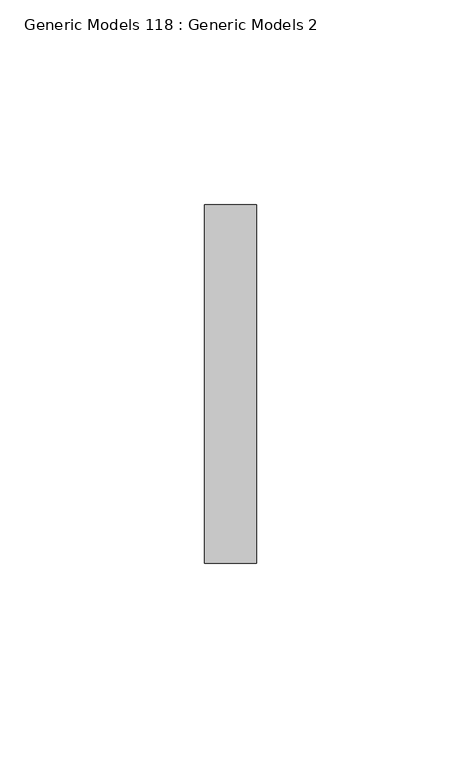
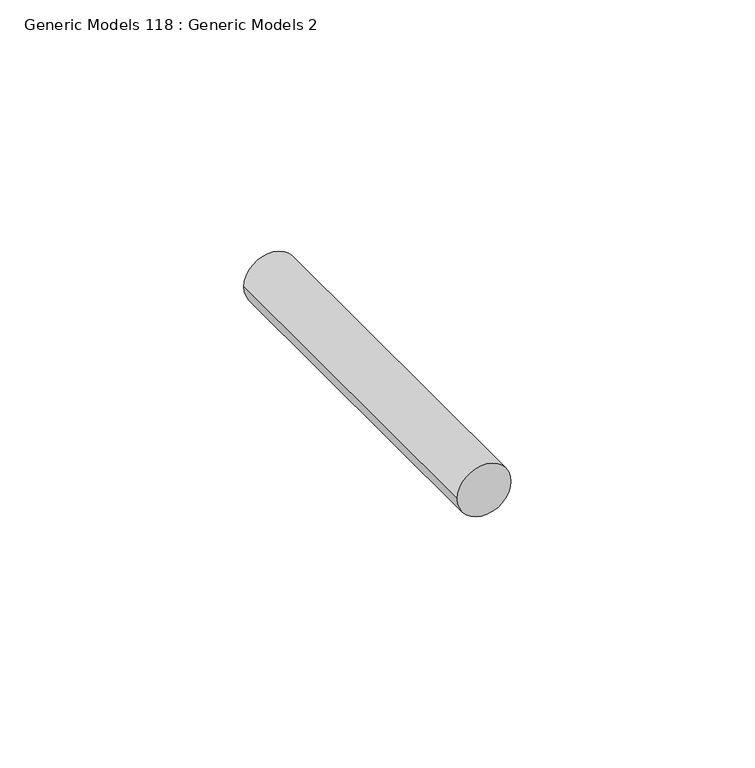
"""IFC4 building model written with IfcOpenShell, lengths in millimetres: proxy geometry, Generic Models 118 : Generic Models 2."""

from ifc_helpers import new_model, si_unit, point, frame, frame_2d, origin, place, context, project, spatial, circle_curve, trimmed, segment, composite_curve, outline, extrude, source, transform, mapped, element, save


def generic_models_118_generic_models_2_6a2263a1(model_context):
    return source(origin(), model_context, "Body", "SweptSolid", [
        extrude(outline(composite_curve([segment(trimmed(circle_curve(frame_2d((38031.9291136, 7128.1828124)), 6.35), [point((38031.9291136, 7121.8328124))], [point((38031.9291136, 7134.5328124))], False, "CARTESIAN"), True, "CONTINUOUS"), segment(trimmed(circle_curve(frame_2d((38031.9291136, 7128.1828124)), 6.35), [point((38031.9291136, 7134.5328124))], [point((38031.9291136, 7121.8328124))], False, "CARTESIAN"), True, "CONTINUOUS")], self_intersect=False)), frame((0.0, 1848.3666731, 0.0), z_axis=(0.0, 1.0, 0.0), x_axis=(0.0, 0.0, 1.0)), (0.0, 0.0, 1.0), 87.551022),
    ])


if __name__ == "__main__":
    model = new_model("IFC4")
    model_context = context("Model", 3, world=origin())
    ifc_project = project(units=[si_unit("LENGTHUNIT", "METRE", prefix="MILLI")], contexts=[model_context])
    site = spatial("IfcSite", under=ifc_project)
    building = spatial("IfcBuilding", under=site)
    placement = place(None, origin())
    generic_models_118_generic_models_2_shape = generic_models_118_generic_models_2_6a2263a1(model_context)
    element("IfcBuildingElementProxy", 1, Name="Generic Models 118 : Generic Models 2", ObjectType="Generic Models 118 : Generic Models 2", at=placement, inside=building, context=model_context, shape_type="MappedRepresentation", body=[
        mapped(generic_models_118_generic_models_2_shape, transform((0.0, 0.0, 0.0), x_axis=(1.0, 0.0, 0.0), y_axis=(0.0, 1.0, 0.0), z_axis=(0.0, 0.0, 1.0))),
    ])
    save(model, "model.ifc")

# Revit data of these elements
# Element 1 (IfcBuildingElementProxy, "Generic Models 118 : Generic Models 2")
#   Materials on its faces: "S.S. LAG BOLT - SEE STRUCT. DWGS"
# Materials
#   "S.S. LAG BOLT - SEE STRUCT. DWGS": class "Generic", colour RGB 120 120 120, transparency 0, Cost = 0
